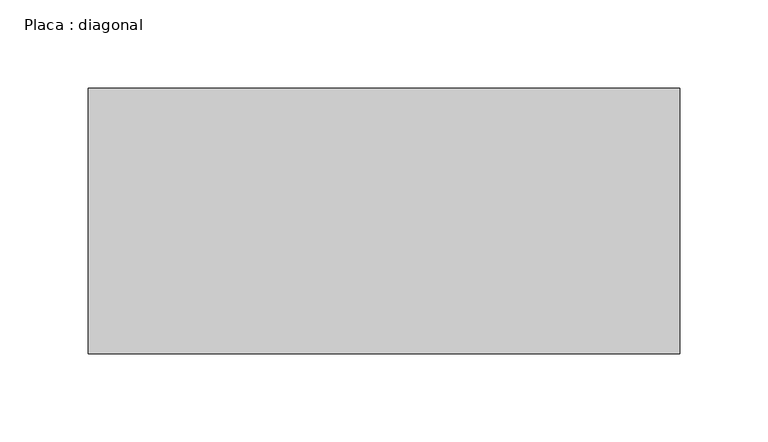
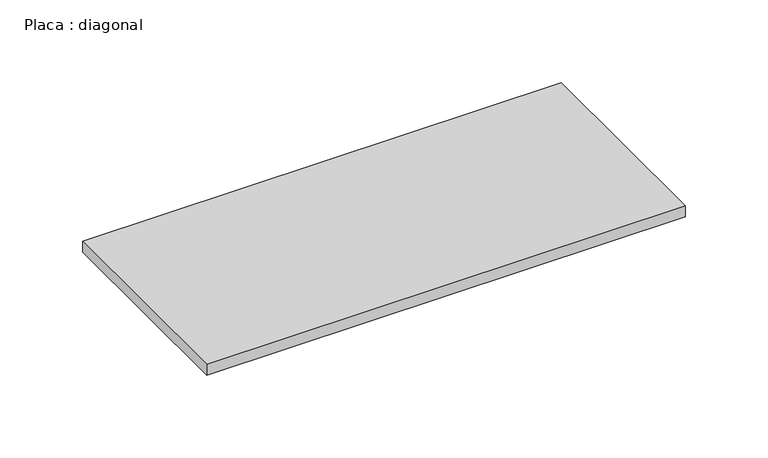
"""IFC4 building model written with IfcOpenShell, lengths in millimetres: beam geometry, Placa : diagonal."""

import ifcopenshell
import ifcopenshell.guid

model = None  # the IFC model being written
_history = None  # IfcOwnerHistory: only IFC2X3 demands one
_inside = {}  # id of a spatial element -> (the spatial element, [elements in it])
_under = {}  # id of a project, library or spatial element -> (it, [spatial elements below it])
_declared = {}  # id of a project -> (the project, [libraries it declares])
_typed = {}  # id of a type object -> (the type object, [elements of that type])
_made_of = {}  # id of a material, layer set ... -> (it, [elements and type objects made of it])


def new_model(schema):
    """Start an empty IFC model of exactly this schema.

    Asked for "IFC4X3", IfcOpenShell would pick the latest addendum, in which some entities
    have other attributes; the version numbers below select the first issue.
    IFC2X3 requires an IfcOwnerHistory on every rooted entity: one is made here for all.
    """
    global model, _history
    if schema == "IFC4X3":
        model = ifcopenshell.file(schema_version=(4, 3, 0, 0))
    else:
        model = ifcopenshell.file(schema=schema)
    _inside.clear()
    _under.clear()
    _declared.clear()
    _typed.clear()
    _made_of.clear()
    _history = None
    if model.schema == "IFC2X3":
        org = make("IfcOrganization", Name="unknown")
        user = make(
            "IfcPersonAndOrganization",
            ThePerson=make("IfcPerson", FamilyName="unknown"),
            TheOrganization=org,
        )
        app = make(
            "IfcApplication",
            ApplicationDeveloper=org,
            Version="unknown",
            ApplicationFullName="unknown",
            ApplicationIdentifier="unknown",
        )
        _history = make(
            "IfcOwnerHistory",
            OwningUser=user,
            OwningApplication=app,
            ChangeAction="ADDED",
            CreationDate=0,
        )
    return model


def make(cls, **values):
    """One entity of the class cls with the attributes given. An attribute that is None is left unset."""
    return model.create_entity(
        cls, **{name: value for name, value in values.items() if value is not None}
    )


def rooted(cls, **values):
    """An entity with a GlobalId (a new one), such as an element, a storey or a relation."""
    return make(cls, GlobalId=ifcopenshell.guid.new(), OwnerHistory=_history, **values)


def si_unit(unit_type, name, prefix=None):
    """IfcSIUnit, for example si_unit("LENGTHUNIT", "METRE", prefix="MILLI")."""
    return make("IfcSIUnit", UnitType=unit_type, Prefix=prefix, Name=name)


def assignment(units):
    """IfcUnitAssignment: the units of a project."""
    return None if units is None else make("IfcUnitAssignment", Units=units)


def point(xyz):
    """IfcCartesianPoint."""
    return None if xyz is None else make("IfcCartesianPoint", Coordinates=xyz)


def direction(xyz):
    """IfcDirection."""
    return None if xyz is None else make("IfcDirection", DirectionRatios=xyz)


def frame(location, z_axis=None, x_axis=None):
    """IfcAxis2Placement3D, a coordinate frame: its origin and axes. An axis left out is left unset."""
    return make(
        "IfcAxis2Placement3D",
        Location=point(location),
        Axis=direction(z_axis),
        RefDirection=direction(x_axis),
    )


def origin():
    """The frame at (0, 0, 0) with its axes left unset."""
    return frame((0.0, 0.0, 0.0))


def place(relative_to, where):
    """IfcLocalPlacement: puts the frame where relative to a parent placement (None: the world)."""
    return make(
        "IfcLocalPlacement", PlacementRelTo=relative_to, RelativePlacement=where
    )


def context(
    kind, dimensions, precision=None, world=None, true_north=None, identifier=None
):
    """IfcGeometricRepresentationContext, for example the 3D "Model" context."""
    return make(
        "IfcGeometricRepresentationContext",
        ContextIdentifier=identifier,
        ContextType=kind,
        CoordinateSpaceDimension=dimensions,
        Precision=precision,
        WorldCoordinateSystem=world,
        TrueNorth=true_north,
    )


def project(units=None, contexts=None):
    """IfcProject with its units and contexts."""
    return rooted(
        "IfcProject",
        Name="project",
        RepresentationContexts=contexts,
        UnitsInContext=assignment(units),
    )


def spatial(cls, under=None, at=None, **own):
    """A site, building, storey or space (cls), placed at a placement, below another one or the project."""
    s = rooted(cls, ObjectPlacement=at, **own)
    if under is not None:
        _under.setdefault(under.id(), (under, []))[1].append(s)
    return s


def polyline(points):
    """IfcPolyline through the points."""
    return make("IfcPolyline", Points=[point(p) for p in points])


def outline(outer, holes=None, kind="AREA"):
    """IfcArbitraryClosedProfileDef: a profile drawn as a closed curve; with holes, ...WithVoids."""
    if holes is None:
        return make("IfcArbitraryClosedProfileDef", ProfileType=kind, OuterCurve=outer)
    return make(
        "IfcArbitraryProfileDefWithVoids",
        ProfileType=kind,
        OuterCurve=outer,
        InnerCurves=holes,
    )


def extrude(swept, where, along, depth):
    """IfcExtrudedAreaSolid: the profile swept, set in the frame where, extruded along a direction by depth."""
    return make(
        "IfcExtrudedAreaSolid",
        SweptArea=swept,
        Position=where,
        ExtrudedDirection=direction(along),
        Depth=depth,
    )


def shape(context_of_items, identifier, shape_type, items):
    """IfcShapeRepresentation: the items that make up one representation, for example the "Body"."""
    return make(
        "IfcShapeRepresentation",
        ContextOfItems=context_of_items,
        RepresentationIdentifier=identifier,
        RepresentationType=shape_type,
        Items=items,
    )


def source(mapping_origin, context_of_items, identifier, shape_type, items):
    """IfcRepresentationMap: a shape defined once, which mapped items show again and again."""
    return make(
        "IfcRepresentationMap",
        MappingOrigin=mapping_origin,
        MappedRepresentation=shape(context_of_items, identifier, shape_type, items),
    )


def transform(
    local_origin,
    x_axis=None,
    y_axis=None,
    z_axis=None,
    scale=None,
    scale2=None,
    scale3=None,
    uniform=True,
):
    """IfcCartesianTransformationOperator3D, or its non-uniform kind. x_axis, y_axis, z_axis: its Axis1, 2, 3."""
    if uniform:
        return make(
            "IfcCartesianTransformationOperator3D",
            Axis1=direction(x_axis),
            Axis2=direction(y_axis),
            LocalOrigin=point(local_origin),
            Scale=scale,
            Axis3=direction(z_axis),
        )
    return make(
        "IfcCartesianTransformationOperator3DnonUniform",
        Axis1=direction(x_axis),
        Axis2=direction(y_axis),
        LocalOrigin=point(local_origin),
        Scale=scale,
        Axis3=direction(z_axis),
        Scale2=scale2,
        Scale3=scale3,
    )


def mapped(mapping_source, mapping_target):
    """IfcMappedItem: shows the shape of a source again, moved by a transform."""
    return make(
        "IfcMappedItem", MappingSource=mapping_source, MappingTarget=mapping_target
    )


def made_of(thing, what):
    """Note that an element or type object is made of a material, layer set ...; save() writes the relation."""
    if what is not None:
        _made_of.setdefault(what.id(), (what, []))[1].append(thing)
    return thing


def element(
    cls,
    number,
    at=None,
    inside=None,
    cuts=None,
    type_object=None,
    material=None,
    context=None,
    identifier="Body",
    shape_type=None,
    held_by="IfcProductDefinitionShape",
    body=None,
    shapes=None,
    **own,
):
    """One element of the class cls, such as IfcWall. Its Tag is "e" and its number.

    at: its placement. inside: the storey or other place that contains it. cuts: it is an
    opening in that element (IfcRelVoidsElement). A single representation is given by context,
    identifier, shape_type and body (its items); several are given by shapes. held_by: the class
    of the entity that holds the representations. save() writes the other relations.
    """
    e = rooted(cls, Tag="e%d" % number, ObjectPlacement=at, **own)
    if body is not None:
        shapes = [shape(context, identifier, shape_type, body)]
    if shapes is not None:
        e.Representation = make(held_by, Representations=shapes)
    if inside is not None:
        _inside.setdefault(inside.id(), (inside, []))[1].append(e)
    if cuts is not None:
        rooted(
            "IfcRelVoidsElement", RelatingBuildingElement=cuts, RelatedOpeningElement=e
        )
    if type_object is not None:
        _typed.setdefault(type_object.id(), (type_object, []))[1].append(e)
    return made_of(e, material)


def aggregate(whole, parts):
    """IfcRelAggregates: a whole, such as a stair, and the parts it consists of."""
    return rooted("IfcRelAggregates", RelatingObject=whole, RelatedObjects=parts)


def save(model, path):
    """Write the relations noted so far, then the file.

    IfcRelAggregates (storeys below a building ...), IfcRelContainedInSpatialStructure (elements
    in a storey), IfcRelDefinesByType, IfcRelAssociatesMaterial and IfcRelDeclares: one each for
    every whole, place, type object, material and project.
    """
    for whole, parts in _under.values():
        aggregate(whole, parts)
    for where, things in _inside.values():
        rooted(
            "IfcRelContainedInSpatialStructure",
            RelatedElements=things,
            RelatingStructure=where,
        )
    for kind, things in _typed.values():
        rooted("IfcRelDefinesByType", RelatedObjects=things, RelatingType=kind)
    for what, things in _made_of.values():
        rooted("IfcRelAssociatesMaterial", RelatedObjects=things, RelatingMaterial=what)
    for by, libraries in _declared.values():
        rooted("IfcRelDeclares", RelatingContext=by, RelatedDefinitions=libraries)
    model.write(path)


def placa_diagonal_d82de291(model_context):
    return source(origin(), model_context, "Body", "SweptSolid", [
        extrude(outline(polyline([(167.0694488, 75.0), (167.0694488, -75.0), (-167.4259573, -75.0), (-167.4259573, 75.0), (167.0694488, 75.0)])), frame((0.0, 0.0, -4.0), z_axis=(0.0, 0.0, 1.0), x_axis=(1.0, 0.0, 0.0)), (0.0, 0.0, 1.0), 8.0),
    ])


if __name__ == "__main__":
    model = new_model("IFC4")
    model_context = context("Model", 3, world=origin())
    ifc_project = project(units=[si_unit("LENGTHUNIT", "METRE", prefix="MILLI")], contexts=[model_context])
    site = spatial("IfcSite", under=ifc_project)
    building = spatial("IfcBuilding", under=site)
    placement = place(None, origin())
    placa_diagonal_shape = placa_diagonal_d82de291(model_context)
    element("IfcBeam", 1, ObjectType="Placa : diagonal", at=placement, inside=building, context=model_context, shape_type="MappedRepresentation", body=[
        mapped(placa_diagonal_shape, transform((0.0, 0.0, 0.0), x_axis=(1.0, 0.0, 0.0), y_axis=(0.0, 1.0, 0.0), z_axis=(0.0, 0.0, 1.0))),
    ])
    save(model, "model.ifc")

# Revit data of these elements
# Type "Placa : diagonal"
#   W = 0
#   Length [instance default] = 1.50 m
#   b = 0.15 m
#   d = 0.008 m
#   A = 0 m²
#   Structural Material [instance default] = Aço, 45-345
# Element 1 (IfcBeam, "Placa : diagonal")
#   Materials on its faces: "Aço, 45-345"
# Materials
#   "Aço, 45-345": class "Metal", colour RGB 247 247 247, transparency 0, Description = "Aço 345 MPa", Cost = 0
